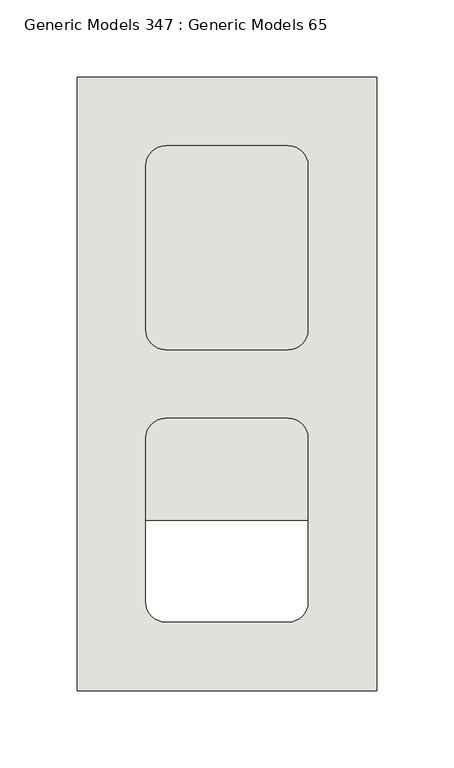
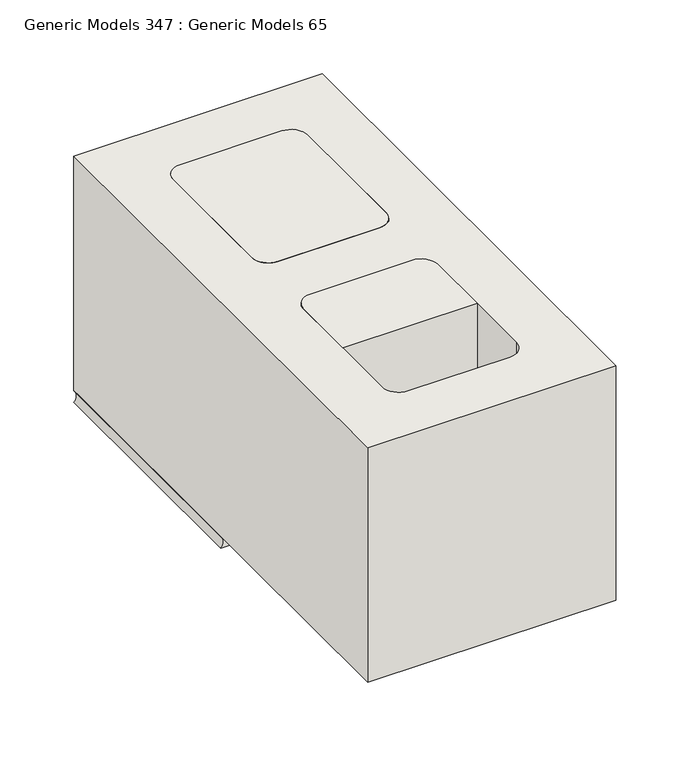
"""IFC4 building model written with IfcOpenShell, lengths in millimetres: wall geometry, Generic Models 347 : Generic Models 65."""

from ifc_helpers import new_model, si_unit, point, frame, frame_2d, origin, place, context, project, spatial, polyline, circle_curve, trimmed, segment, composite_curve, outline, extrude, source, transform, mapped, element, save
from ifc_brep_helpers import plane_surface, revolved_surface, advanced_brep


def generic_models_347_generic_models_65_8ecf3a24(model_context):
    return source(origin(), model_context, "Body", "SolidModel", [
        advanced_brep(
        [(430198.2125, 503.2375, 1025.525), (430004.5375, 503.2375, 1025.525), (430004.5375, 503.2375, 1016.0), (430198.2125, 503.2375, 1016.0), (430198.2125, 701.675, 1025.525), (430198.2125, 701.675, 1016.0), (430004.5375, 701.675, 1016.0), (430004.5375, 701.675, 1025.525), (430153.7625, 538.1625, 1025.525), (430141.0625, 525.4625, 1025.525), (430061.6875, 525.4625, 1025.525), (430048.9875, 538.1625, 1025.525), (430048.9875, 644.525, 1025.525), (430061.6875, 657.225, 1025.525), (430141.0625, 657.225, 1025.525), (430153.7625, 644.525, 1025.525), (430141.0625, 525.4625, 1016.0), (430153.7625, 538.1625, 1016.0), (430061.6875, 525.4625, 1016.0), (430048.9875, 538.1625, 1016.0), (430048.9875, 644.525, 1016.0), (430061.6875, 657.225, 1016.0), (430141.0625, 657.225, 1016.0), (430153.7625, 644.525, 1016.0)],
        [
            (0, 1),
            (1, 2, circle_curve(frame((429999.6545028, 503.2375, 1020.7625), z_axis=(0.0, 1.0, 0.0), x_axis=(1.0, 0.0, 0.0)), 6.8209287)),
            (2, 3),
            (3, 0, circle_curve(frame((430203.0954972, 503.2375, 1020.7625), z_axis=(0.0, 1.0, 0.0), x_axis=(-1.0, 0.0, 0.0)), 6.8209287)),
            (4, 5, circle_curve(frame((430203.0954972, 701.675, 1020.7625), z_axis=(0.0, -1.0, 0.0), x_axis=(-1.0, 0.0, 0.0)), 6.8209287)),
            (5, 6),
            (6, 7, circle_curve(frame((429999.6545028, 701.675, 1020.7625), z_axis=(0.0, -1.0, 0.0), x_axis=(1.0, 0.0, 0.0)), 6.8209287)),
            (7, 4),
            (0, 4),
            (7, 1),
            (8, 9, circle_curve(frame((430141.0625, 538.1625, 1025.525), z_axis=(0.0, 0.0, -1.0), x_axis=(-1.0, 0.0, 0.0)), 12.7)),
            (9, 10),
            (10, 11, circle_curve(frame((430061.6875, 538.1625, 1025.525), z_axis=(0.0, 0.0, -1.0), x_axis=(-1.0, 0.0, 0.0)), 12.7)),
            (11, 12),
            (12, 13, circle_curve(frame((430061.6875, 644.525, 1025.525), z_axis=(0.0, 0.0, -1.0), x_axis=(-1.0, 0.0, 0.0)), 12.7)),
            (13, 14),
            (14, 15, circle_curve(frame((430141.0625, 644.525, 1025.525), z_axis=(0.0, 0.0, -1.0), x_axis=(-1.0, 0.0, 0.0)), 12.7)),
            (15, 8),
            (16, 9),
            (8, 17),
            (17, 16, circle_curve(frame((430141.0625, 538.1625, 1016.0), z_axis=(0.0, 0.0, -1.0), x_axis=(-1.0, 0.0, 0.0)), 12.7)),
            (16, 18),
            (18, 10),
            (18, 19, circle_curve(frame((430061.6875, 538.1625, 1016.0), z_axis=(0.0, 0.0, -1.0), x_axis=(-1.0, 0.0, 0.0)), 12.7)),
            (19, 11),
            (19, 20),
            (20, 12),
            (20, 21, circle_curve(frame((430061.6875, 644.525, 1016.0), z_axis=(0.0, 0.0, -1.0), x_axis=(-1.0, 0.0, 0.0)), 12.7)),
            (21, 13),
            (21, 22),
            (22, 14),
            (22, 23, circle_curve(frame((430141.0625, 644.525, 1016.0), z_axis=(0.0, 0.0, -1.0), x_axis=(-1.0, 0.0, 0.0)), 12.7)),
            (23, 15),
            (23, 17),
            (6, 2),
            (5, 3),
        ],
        [
            plane_surface(frame((430101.375, 503.2375, 1025.921875), z_axis=(0.0, -1.0, 0.0), x_axis=(0.0, 0.0, 1.0))),
            plane_surface(frame((430101.375, 701.675, 1025.921875), z_axis=(0.0, 1.0, 0.0), x_axis=(0.0, 0.0, 1.0))),
            plane_surface(frame((430198.2125, 503.2375, 1025.525), z_axis=(0.0, 0.0, 1.0), x_axis=(0.0, 1.0, 0.0))),
            revolved_surface(polyline([(430128.3625, 538.1625, 1025.525), (430128.3625, 538.1625, 1016.0)]), (430141.0625, 538.1625, 1209.675), (0.0, 0.0, 1.0)),
            plane_surface(frame((430061.6875, 525.4625, 1209.675), z_axis=(0.0, 1.0, 0.0), x_axis=(0.0, 0.0, -1.0))),
            revolved_surface(polyline([(430048.9875, 538.1625, 1025.525), (430048.9875, 538.1625, 1016.0)]), (430061.6875, 538.1625, 1209.675), (0.0, 0.0, 1.0)),
            plane_surface(frame((430048.9875, 644.525, 1209.675), z_axis=(1.0, 0.0, 0.0), x_axis=(0.0, 0.0, -1.0))),
            revolved_surface(polyline([(430048.9875, 644.525, 1025.525), (430048.9875, 644.525, 1016.0)]), (430061.6875, 644.525, 1209.675), (0.0, 0.0, 1.0)),
            plane_surface(frame((430141.0625, 657.225, 1209.675), z_axis=(0.0, -1.0, 0.0), x_axis=(0.0, 0.0, -1.0))),
            revolved_surface(polyline([(430128.3625, 644.525, 1025.525), (430128.3625, 644.525, 1016.0)]), (430141.0625, 644.525, 1209.675), (0.0, 0.0, 1.0)),
            plane_surface(frame((430153.7625, 538.1625, 1209.675), z_axis=(-1.0, 0.0, 0.0), x_axis=(0.0, 0.0, -1.0))),
            revolved_surface(polyline([(430006.4754315, 701.675, 1020.7625), (430006.4754315, 503.2375, 1020.7625)]), (429999.6545028, 503.2375, 1020.7625), (0.0, 1.0, 0.0)),
            plane_surface(frame((430004.5375, 503.2375, 1016.0), z_axis=(0.0, 0.0, -1.0), x_axis=(0.0, 1.0, 0.0))),
            revolved_surface(polyline([(430196.2745685, 701.675, 1020.7625), (430196.2745685, 503.2375, 1020.7625)]), (430203.0954972, 503.2375, 1020.7625), (0.0, 1.0, 0.0)),
        ],
        [
            (0, [[1, 2, 3, 4]]),
            (1, [[5, 6, 7, 8]]),
            (2, [[-1, 9, -8, 10], [11, 12, 13, 14, 15, 16, 17, 18]]),
            (3, [[19, -11, 20, 21]]),
            (4, [[-19, 22, 23, -12]]),
            (5, [[-23, 24, 25, -13]]),
            (6, [[-25, 26, 27, -14]]),
            (7, [[-27, 28, 29, -15]]),
            (8, [[-29, 30, 31, -16]]),
            (9, [[-31, 32, 33, -17]]),
            (10, [[-33, 34, -20, -18]]),
            (11, [[-2, -10, -7, 35]]),
            (12, [[-3, -35, -6, 36], [-21, -34, -32, -30, -28, -26, -24, -22]]),
            (13, [[-4, -36, -5, -9]]),
        ],
    ),
        extrude(outline(composite_curve([segment(trimmed(circle_curve(frame_2d((430141.0625, 538.1625)), 12.7), [point((430153.7625, 538.1625))], [point((430141.0625, 525.4625))], False, "CARTESIAN"), True, "CONTINUOUS"), segment(polyline([(430141.0625, 525.4625), (430061.6875, 525.4625)]), True, "CONTINUOUS"), segment(trimmed(circle_curve(frame_2d((430061.6875, 538.1625)), 12.7), [point((430061.6875, 525.4625))], [point((430048.9875, 538.1625))], False, "CARTESIAN"), True, "CONTINUOUS"), segment(polyline([(430048.9875, 538.1625), (430048.9875, 644.525)]), True, "CONTINUOUS"), segment(trimmed(circle_curve(frame_2d((430061.6875, 644.525)), 12.7), [point((430048.9875, 644.525))], [point((430061.6875, 657.225))], False, "CARTESIAN"), True, "CONTINUOUS"), segment(polyline([(430061.6875, 657.225), (430141.0625, 657.225)]), True, "CONTINUOUS"), segment(trimmed(circle_curve(frame_2d((430141.0625, 644.525)), 12.7), [point((430141.0625, 657.225))], [point((430153.7625, 644.525))], False, "CARTESIAN"), True, "CONTINUOUS"), segment(polyline([(430153.7625, 644.525), (430153.7625, 538.1625)]), True, "CONTINUOUS")], self_intersect=False)), frame((0.0, 0.0, 1016.0), z_axis=(0.0, 0.0, 1.0), x_axis=(1.0, 0.0, 0.0)), (0.0, 0.0, 1.0), 203.2),
        extrude(outline(composite_curve([segment(trimmed(circle_curve(frame_2d((430061.6875, 468.3125)), 12.7), [point((430048.9875, 468.3125))], [point((430061.6875, 481.0125))], False, "CARTESIAN"), True, "CONTINUOUS"), segment(polyline([(430061.6875, 481.0125), (430141.0625, 481.0125)]), True, "CONTINUOUS"), segment(trimmed(circle_curve(frame_2d((430141.0625, 468.3125)), 12.7), [point((430141.0625, 481.0125))], [point((430153.7625, 468.3125))], False, "CARTESIAN"), True, "CONTINUOUS"), segment(polyline([(430153.7625, 468.3125), (430153.7625, 415.13125), (430048.9875, 415.13125), (430048.9875, 468.3125)]), True, "CONTINUOUS")], self_intersect=False)), frame((0.0, 0.0, 1016.0), z_axis=(0.0, 0.0, 1.0), x_axis=(1.0, 0.0, 0.0)), (0.0, 0.0, 1.0), 203.2),
        extrude(outline(polyline([(430198.2125, 304.8), (430004.5375, 304.8), (430004.5375, 701.675), (430198.2125, 701.675), (430198.2125, 304.8)]), holes=[composite_curve([segment(polyline([(430153.7625, 538.1625), (430153.7625, 644.525)]), True, "CONTINUOUS"), segment(trimmed(circle_curve(frame_2d((430141.0625, 644.525)), 12.7), [point((430153.7625, 644.525))], [point((430141.0625, 657.225))], True, "CARTESIAN"), True, "CONTINUOUS"), segment(polyline([(430141.0625, 657.225), (430061.6875, 657.225)]), True, "CONTINUOUS"), segment(trimmed(circle_curve(frame_2d((430061.6875, 644.525)), 12.7), [point((430061.6875, 657.225))], [point((430048.9875, 644.525))], True, "CARTESIAN"), True, "CONTINUOUS"), segment(polyline([(430048.9875, 644.525), (430048.9875, 538.1625)]), True, "CONTINUOUS"), segment(trimmed(circle_curve(frame_2d((430061.6875, 538.1625)), 12.7), [point((430048.9875, 538.1625))], [point((430061.6875, 525.4625))], True, "CARTESIAN"), True, "CONTINUOUS"), segment(polyline([(430061.6875, 525.4625), (430141.0625, 525.4625)]), True, "CONTINUOUS"), segment(trimmed(circle_curve(frame_2d((430141.0625, 538.1625)), 12.7), [point((430141.0625, 525.4625))], [point((430153.7625, 538.1625))], True, "CARTESIAN"), True, "CONTINUOUS")], self_intersect=False), composite_curve([segment(polyline([(430048.9875, 468.3125), (430048.9875, 361.95)]), True, "CONTINUOUS"), segment(trimmed(circle_curve(frame_2d((430061.6875, 361.95)), 12.7), [point((430048.9875, 361.95))], [point((430061.6875, 349.25))], True, "CARTESIAN"), True, "CONTINUOUS"), segment(polyline([(430061.6875, 349.25), (430141.0625, 349.25)]), True, "CONTINUOUS"), segment(trimmed(circle_curve(frame_2d((430141.0625, 361.95)), 12.7), [point((430141.0625, 349.25))], [point((430153.7625, 361.95))], True, "CARTESIAN"), True, "CONTINUOUS"), segment(polyline([(430153.7625, 361.95), (430153.7625, 468.3125)]), True, "CONTINUOUS"), segment(trimmed(circle_curve(frame_2d((430141.0625, 468.3125)), 12.7), [point((430153.7625, 468.3125))], [point((430141.0625, 481.0125))], True, "CARTESIAN"), True, "CONTINUOUS"), segment(polyline([(430141.0625, 481.0125), (430061.6875, 481.0125)]), True, "CONTINUOUS"), segment(trimmed(circle_curve(frame_2d((430061.6875, 468.3125)), 12.7), [point((430061.6875, 481.0125))], [point((430048.9875, 468.3125))], True, "CARTESIAN"), True, "CONTINUOUS")], self_intersect=False)]), frame((0.0, 0.0, 1025.525), z_axis=(0.0, 0.0, 1.0), x_axis=(1.0, 0.0, 0.0)), (0.0, 0.0, 1.0), 193.675),
    ])


if __name__ == "__main__":
    model = new_model("IFC4")
    model_context = context("Model", 3, world=origin())
    ifc_project = project(units=[si_unit("LENGTHUNIT", "METRE", prefix="MILLI")], contexts=[model_context])
    site = spatial("IfcSite", under=ifc_project)
    building = spatial("IfcBuilding", under=site)
    placement = place(None, origin())
    generic_models_347_generic_models_65_shape = generic_models_347_generic_models_65_8ecf3a24(model_context)
    element("IfcWall", 1, ObjectType="Generic Models 347 : Generic Models 65", at=placement, inside=building, context=model_context, shape_type="MappedRepresentation", body=[
        mapped(generic_models_347_generic_models_65_shape, transform((0.0, 0.0, 0.0), x_axis=(1.0, 0.0, 0.0), y_axis=(0.0, 1.0, 0.0), z_axis=(0.0, 0.0, 1.0))),
    ])
    save(model, "model.ifc")

# Revit data of these elements
# Element 1 (IfcWall, "Generic Models 347 : Generic Models 65")
#   Materials on its faces: "CMU (SEE 'WALL TAG' FOR SIZE)", "FILL CORE IF APPLICABLE - SEE STRUCTURAL DWGS FOR DETAILS", "MORTAR JOINT"
# Materials
#   "CMU (SEE 'WALL TAG' FOR SIZE)": class "Masonry", colour RGB 203 203 199, transparency 0, Description = "Concrete masonry units", Cost = 0
#   "FILL CORE IF APPLICABLE - SEE STRUCTURAL DWGS FOR DETAILS": class "Generic", colour RGB 170 170 170, transparency 0, Cost = 0
#   "MORTAR JOINT": class "Generic", colour RGB 120 120 120, transparency 0, Cost = 0
